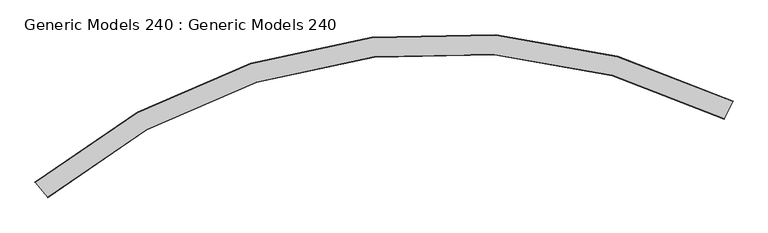
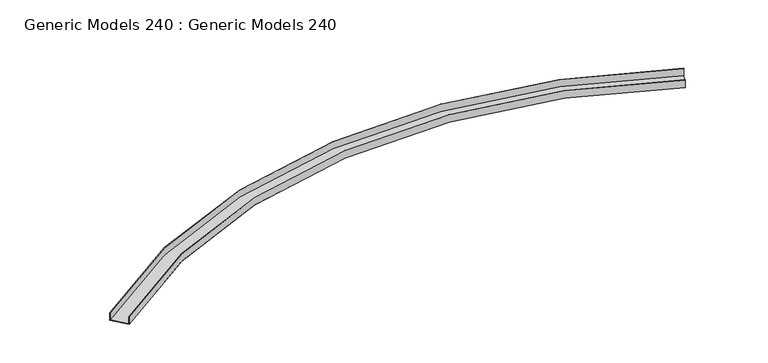
"""IFC4 building model written with IfcOpenShell, lengths in millimetres: proxy geometry, Generic Models 240 : Generic Models 240."""

from ifc_helpers import new_model, si_unit, frame, origin, place, context, project, spatial, polyline, circle_curve, source, transform, mapped, element, save
from ifc_brep_helpers import plane_surface, cylinder_surface, revolved_surface, advanced_brep


def generic_models_240_generic_models_240_95c696e8(model_context):
    return source(origin(), model_context, "Body", "AdvancedBrep", [
        advanced_brep(
        [(485.1422677, -22517.2153765, 0.0), (485.1422677, -22517.2153765, 41.275), (484.4296516, -22518.6339443, 41.275), (484.4296516, -22518.6339443, 1.5875), (444.5231527, -22598.0737413, 1.5875), (444.5231527, -22598.0737413, 41.275), (443.8105367, -22599.4923091, 41.275), (443.8105367, -22599.4923091, 0.0), (-2715.400226, -22889.127437, 0.0), (-2656.3029741, -22959.7342387, 0.0), (-2656.3029741, -22959.7342387, 41.275), (-2657.3218922, -22958.51688, 41.275), (-2657.3218922, -22958.51688, 1.5875), (-2714.3813078, -22890.3447957, 1.5875), (-2714.3813078, -22890.3447957, 41.275), (-2715.400226, -22889.127437, 41.275)],
        [
            (0, 1),
            (1, 2),
            (2, 3),
            (3, 4),
            (4, 5),
            (5, 6),
            (6, 7),
            (7, 0),
            (8, 9),
            (9, 10),
            (10, 11),
            (11, 12),
            (12, 13),
            (13, 14),
            (14, 15),
            (15, 8),
            (15, 1, circle_curve(frame((-832.04683, -25139.2753781, 41.275), z_axis=(0.0, 0.0, -1.0), x_axis=(0.44889200092737946, 0.8935860179654858, 0.0)), 2934.3118053)),
            (0, 8, circle_curve(frame((-832.04683, -25139.2753781, 0.0), z_axis=(0.0, 0.0, 1.0), x_axis=(0.44889200092737946, 0.8935860179654858, 0.0)), 2934.3118053)),
            (14, 2, circle_curve(frame((-832.04683, -25139.2753781, 41.275), z_axis=(0.0, 0.0, -1.0), x_axis=(0.44889200092737946, 0.8935860179654858, 0.0)), 2932.7243053)),
            (13, 3, circle_curve(frame((-832.04683, -25139.2753781, 1.5875), z_axis=(0.0, 0.0, -1.0), x_axis=(0.44889200092737946, 0.8935860179654858, 0.0)), 2932.7243053)),
            (12, 4, circle_curve(frame((-832.04683, -25139.2753781, 1.5875), z_axis=(0.0, 0.0, -1.0), x_axis=(0.44889200092737946, 0.8935860179654858, 0.0)), 2843.8243053)),
            (11, 5, circle_curve(frame((-832.04683, -25139.2753781, 41.275), z_axis=(0.0, 0.0, -1.0), x_axis=(0.44889200092737946, 0.8935860179654858, 0.0)), 2843.8243053)),
            (10, 6, circle_curve(frame((-832.04683, -25139.2753781, 41.275), z_axis=(0.0, 0.0, -1.0), x_axis=(0.44889200092737946, 0.8935860179654858, 0.0)), 2842.2368053)),
            (9, 7, circle_curve(frame((-832.04683, -25139.2753781, 0.0), z_axis=(0.0, 0.0, -1.0), x_axis=(0.44889200092737946, 0.8935860179654858, 0.0)), 2842.2368053)),
        ],
        [
            plane_surface(frame((536.1759889, -22415.6251953, 0.0), z_axis=(0.8935860179654859, -0.4488920009273796, 0.0), x_axis=(0.0, 0.0, 1.0))),
            plane_surface(frame((-2788.3696518, -22801.9467711, 0.0), z_axis=(-0.7668400941499618, -0.6418381961242863, 0.0), x_axis=(0.0, 0.0, 1.0))),
            cylinder_surface(frame((-832.04683, -25139.2753781, 0.0), z_axis=(0.0, 0.0, 1.0), x_axis=(0.44889200092737946, 0.8935860179654858, 0.0)), 2934.3118053),
            plane_surface(frame((-832.04683, -25139.2753781, 41.275), z_axis=(0.0, 0.0, 1.0000000000000002), x_axis=(0.4488920009273795, 0.8935860179654859, 0.0))),
            revolved_surface(polyline([(484.4296515744759, -22518.633944336376, 41.275), (484.4296515744759, -22518.633944336376, 1.5875)]), (-832.04683, -25139.2753781, 0.0), (0.0, 0.0, 1.0)),
            plane_surface(frame((-832.04683, -25139.2753781, 1.5875), z_axis=(0.0, 0.0, 1.0000000000000002), x_axis=(0.4488920009273795, 0.8935860179654859, 0.0))),
            cylinder_surface(frame((-832.04683, -25139.2753781, 0.0), z_axis=(0.0, 0.0, 1.0), x_axis=(0.44889200092737946, 0.8935860179654858, 0.0)), 2843.8243053),
            revolved_surface(polyline([(443.8105366405596, -22599.49230913703, 41.275), (443.8105366405596, -22599.49230913703, 0.0)]), (-832.04683, -25139.2753781, 0.0), (0.0, 0.0, 1.0)),
            plane_surface(frame((-832.04683, -25139.2753781, 0.0), z_axis=(0.0, 0.0, -1.0000000000000002), x_axis=(0.4488920009273795, 0.8935860179654859, 0.0))),
        ],
        [
            (0, [[1, 2, 3, 4, 5, 6, 7, 8]]),
            (1, [[9, 10, 11, 12, 13, 14, 15, 16]]),
            (2, [[17, -1, 18, -16]]),
            (3, [[19, -2, -17, -15]]),
            (4, [[20, -3, -19, -14]]),
            (5, [[21, -4, -20, -13]]),
            (6, [[22, -5, -21, -12]]),
            (3, [[23, -6, -22, -11]]),
            (7, [[24, -7, -23, -10]]),
            (8, [[-18, -8, -24, -9]]),
        ],
    ),
    ])


if __name__ == "__main__":
    model = new_model("IFC4")
    model_context = context("Model", 3, world=origin())
    ifc_project = project(units=[si_unit("LENGTHUNIT", "METRE", prefix="MILLI")], contexts=[model_context])
    site = spatial("IfcSite", under=ifc_project)
    building = spatial("IfcBuilding", under=site)
    placement = place(None, origin())
    generic_models_240_generic_models_240_shape = generic_models_240_generic_models_240_95c696e8(model_context)
    element("IfcBuildingElementProxy", 1, Name="Generic Models 240 : Generic Models 240", ObjectType="Generic Models 240 : Generic Models 240", at=placement, inside=building, context=model_context, shape_type="MappedRepresentation", body=[
        mapped(generic_models_240_generic_models_240_shape, transform((0.0, 0.0, 0.0), x_axis=(1.0, 0.0, 0.0), y_axis=(0.0, 1.0, 0.0), z_axis=(0.0, 0.0, 1.0))),
    ])
    save(model, "model.ifc")

# Revit data of these elements
# Element 1 (IfcBuildingElementProxy, "Generic Models 240 : Generic Models 240")
#   Materials on its faces: "METAL STUDS WITH CURVE TRACKS"
# Materials
#   "METAL STUDS WITH CURVE TRACKS": class "Unassigned", colour RGB 210 209 208, transparency 0, Keynote = "M05121300.02", Cost = 0
